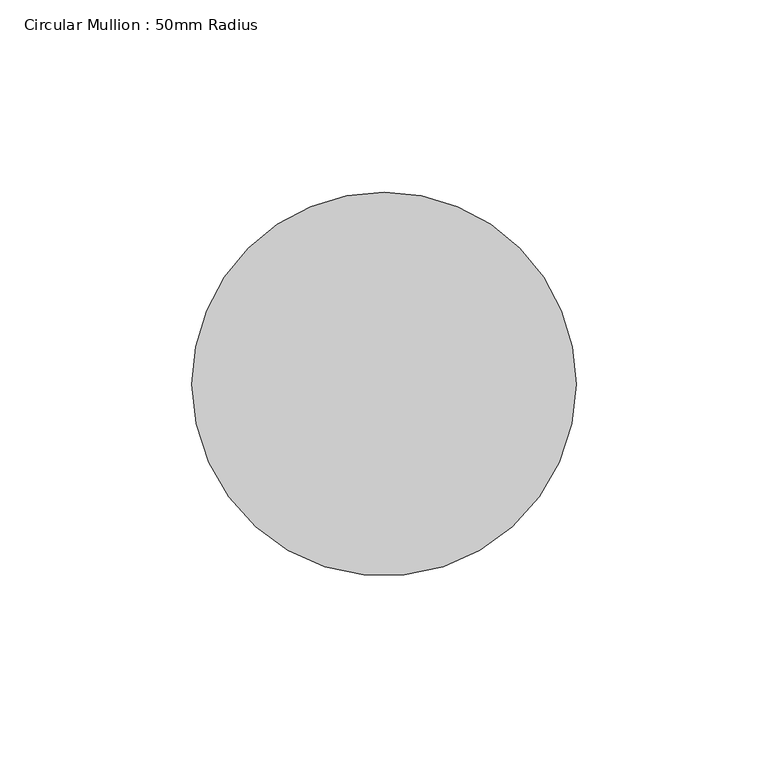
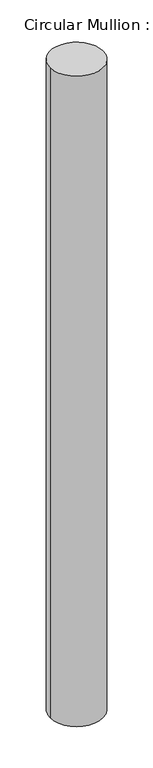
"""IFC4 building model written with IfcOpenShell, lengths in millimetres: member geometry, Circular Mullion : 50mm Radius."""

from ifc_helpers import new_model, si_unit, frame, origin, place, context, project, spatial, ellipse_curve, source, transform, mapped, element, save
from ifc_brep_helpers import plane_surface, cylinder_surface, advanced_brep


def circular_mullion_50mm_radius_e49311c1(model_context):
    return source(origin(), model_context, "Body", "AdvancedBrep", [
        advanced_brep(
        [(-100.0, 0.0, 0.9503605), (0.0, 0.0, 0.0), (0.0, 0.0, -1300.059613), (-100.0, 0.0, -1300.9523468)],
        [
            (0, 1, ellipse_curve(frame((-50.0, 0.0, 0.4751802), z_axis=(-0.009501703276228193, -0.01760331765598219, -0.9997999004012519), x_axis=(-0.47489562976836275, -0.8798147428119533, 0.020003978545446683)), 50.010007, 50.0)),
            (1, 2),
            (2, 3, ellipse_curve(frame((-50.0, 0.0, -1300.5059799), z_axis=(-0.008925761184937615, -0.01653629932361647, 0.9998234252066458), x_axis=(0.47490680383155204, 0.8798354444249499, 0.018791445076169994)), 50.0088303, 50.0)),
            (3, 0),
            (1, 0, ellipse_curve(frame((-50.0, 0.0, 0.4751802), z_axis=(-0.009501703276228193, -0.01760331765598219, -0.9997999004012519), x_axis=(-0.47489562976836275, -0.8798147428119533, 0.020003978545446683)), 50.010007, 50.0)),
            (3, 2, ellipse_curve(frame((-50.0, 0.0, -1300.5059799), z_axis=(-0.008925761184937615, -0.01653629932361647, 0.9998234252066458), x_axis=(0.47490680383155204, 0.8798354444249499, 0.018791445076169994)), 50.0088303, 50.0)),
        ],
        [
            cylinder_surface(frame((-50.0, 0.0, 0.0), z_axis=(0.0, 0.0, 1.0), x_axis=(1.0, 0.0, 0.0)), 50.0),
            plane_surface(frame((-268.2212046, 144.7771578, 0.0), z_axis=(0.009501703276228193, 0.01760331765598219, 0.9997999004012519), x_axis=(0.4748956297683628, 0.8798147428119532, -0.020003978545451898))),
            plane_surface(frame((-268.2212046, 144.7771578, -1300.059613), z_axis=(0.008925761184937616, 0.016536299323616475, -0.999823425206646), x_axis=(0.474906803831552, 0.87983544442495, 0.0187914450761717))),
        ],
        [
            (0, [[1, 2, 3, 4]]),
            (0, [[5, -4, 6, -2]]),
            (1, [[-1, -5]]),
            (2, [[-6, -3]]),
        ],
    ),
    ])


if __name__ == "__main__":
    model = new_model("IFC4")
    model_context = context("Model", 3, world=origin())
    ifc_project = project(units=[si_unit("LENGTHUNIT", "METRE", prefix="MILLI")], contexts=[model_context])
    site = spatial("IfcSite", under=ifc_project)
    building = spatial("IfcBuilding", under=site)
    placement = place(None, origin())
    circular_mullion_50mm_radius_shape = circular_mullion_50mm_radius_e49311c1(model_context)
    element("IfcMember", 1, ObjectType="Circular Mullion : 50mm Radius", at=placement, inside=building, context=model_context, shape_type="MappedRepresentation", body=[
        mapped(circular_mullion_50mm_radius_shape, transform((0.0, 0.0, 0.0), x_axis=(1.0, 0.0, 0.0), y_axis=(0.0, 1.0, 0.0), z_axis=(0.0, 0.0, 1.0))),
    ])
    save(model, "model.ifc")

# Revit data of these elements
# Type "Circular Mullion : 50mm Radius"
#   built-in parameter 1007350 = 0.164042 (stored number, unit not read)
# Element 1 (IfcMember, "Circular Mullion : 50mm Radius")
#   Materials on its faces: "Aluminium"
# Materials
#   "Aluminium": class "Metal", colour RGB 247 247 247, transparency 0, Description = "Aluminium 6061", Cost = 0
